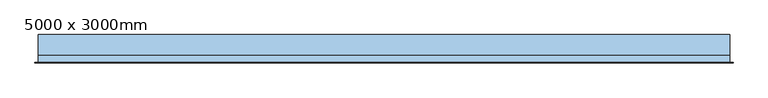
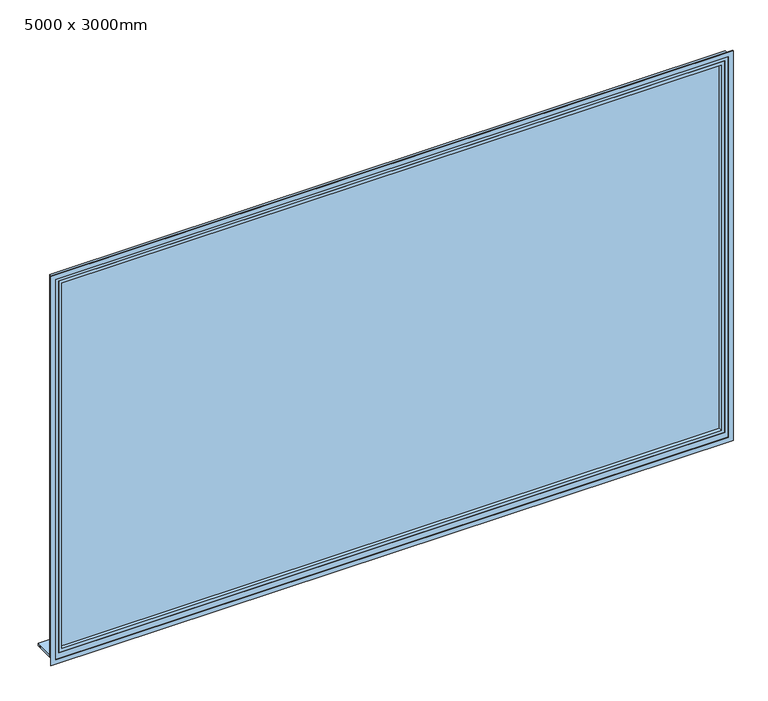
"""IFC4 building model written with IfcOpenShell, lengths in millimetres: window geometry, Ventana simple fija con cubrejuntas interior : 5000 x 3000mm."""

from ifc_helpers import new_model, si_unit, frame, origin, place, context, project, spatial, polyline, outline, extrude, faceted_brep, source, transform, mapped, element, save


def window_5000_x_3000mm_49c9fe68(model_context):
    return source(origin(), model_context, "Body", "SolidModel", [
        extrude(outline(polyline([(125.0, 920.0), (125.0, 900.0), (105.0, 900.0), (105.0, 910.0), (95.0, 910.0), (95.0, 900.0), (-25.0, 900.0), (-25.0, 920.0), (125.0, 920.0)])), frame((-2500.0, 0.0, 0.0), z_axis=(1.0, 0.0, 0.0), x_axis=(0.0, 1.0, 0.0)), (0.0, 0.0, 1.0), 5000.0),
        extrude(outline(polyline([(-2455.0, -49.0), (-2455.0, -35.0), (2455.0, -35.0), (2455.0, -49.0), (-2455.0, -49.0)])), frame((0.0, 0.0, 965.0), z_axis=(0.0, 0.0, 1.0), x_axis=(1.0, 0.0, 0.0)), (0.0, 0.0, 1.0), 2890.0),
        extrude(outline(polyline([(3865.0, -2465.0), (955.0, -2465.0), (955.0, 2465.0), (3865.0, 2465.0), (3865.0, -2465.0)]), holes=[polyline([(3840.0, 2440.0), (980.0, 2440.0), (980.0, -2440.0), (3840.0, -2440.0), (3840.0, 2440.0)])]), frame((0.0, -75.0, 0.0), z_axis=(0.0, 1.0, 0.0), x_axis=(0.0, 0.0, 1.0)), (0.0, 0.0, 1.0), 26.0),
        faceted_brep([(2500.0, -25.0, 3900.0), (2500.0, -75.0, 3900.0), (2500.0, -75.0, 900.0), (2500.0, -25.0, 900.0), (-2500.0, -75.0, 3900.0), (-2500.0, -75.0, 900.0), (-2465.0, -75.0, 3865.0), (2465.0, -75.0, 3865.0), (2465.0, -75.0, 955.0), (-2465.0, -75.0, 955.0), (-2500.0, -25.0, 900.0), (-2500.0, -25.0, 3900.0), (2440.0, -25.0, 3840.0), (-2440.0, -25.0, 3840.0), (-2440.0, -25.0, 980.0), (2440.0, -25.0, 980.0), (2440.0, -35.0, 3840.0), (2440.0, -35.0, 980.0), (-2440.0, -35.0, 980.0), (2465.0, -35.0, 3865.0), (-2465.0, -35.0, 3865.0), (-2465.0, -35.0, 955.0), (2465.0, -35.0, 955.0), (-2440.0, -35.0, 3840.0)], [[[0, 1, 2, 3]], [[2, 1, 4, 5], [6, 7, 8, 9]], [[5, 10, 3, 2]], [[10, 11, 0, 3], [12, 13, 14, 15]], [[16, 12, 15, 17]], [[17, 15, 14, 18]], [[19, 20, 21, 22], [23, 16, 17, 18]], [[7, 19, 22, 8]], [[8, 22, 21, 9]], [[13, 23, 18, 14]], [[20, 6, 9, 21]], [[4, 11, 10, 5]], [[11, 4, 1, 0]], [[23, 13, 12, 16]], [[6, 20, 19, 7]]]),
        extrude(outline(polyline([(3925.0, -2525.0), (875.0, -2525.0), (875.0, 2525.0), (3925.0, 2525.0), (3925.0, -2525.0)]), holes=[polyline([(3890.0, 2490.0), (910.0, 2490.0), (910.0, -2490.0), (3890.0, -2490.0), (3890.0, 2490.0)])]), frame((0.0, -80.0, 0.0), z_axis=(0.0, 1.0, 0.0), x_axis=(0.0, 0.0, 1.0)), (0.0, 0.0, 1.0), 5.0),
    ])


if __name__ == "__main__":
    model = new_model("IFC4")
    model_context = context("Model", 3, world=origin())
    ifc_project = project(units=[si_unit("LENGTHUNIT", "METRE", prefix="MILLI")], contexts=[model_context])
    site = spatial("IfcSite", under=ifc_project)
    building = spatial("IfcBuilding", under=site)
    placement = place(None, origin())
    window_5000_x_3000mm_shape = window_5000_x_3000mm_49c9fe68(model_context)
    element("IfcWindow", 1, ObjectType="Ventana simple fija con cubrejuntas interior : 5000 x 3000mm", at=placement, inside=building, context=model_context, shape_type="MappedRepresentation", body=[
        mapped(window_5000_x_3000mm_shape, transform((0.0, 0.0, 0.0), x_axis=(1.0, 0.0, 0.0), y_axis=(0.0, 1.0, 0.0), z_axis=(0.0, 0.0, 1.0))),
    ])
    save(model, "model.ifc")

# Revit data of these elements
# Type "Ventana simple fija con cubrejuntas interior : 5000 x 3000mm"
#   Type Mark = "41"
#   Construction Type Id = "GSP4R"
#   Analytic Construction = "1/8 en cristalera simple Pilkington"
#   Grosor de pared [instance default] = 0.20 m
#   W1 = 4.88 m
#   Visual Light Transmittance = 0.9
#   Anchura de cubrejuntas = 0.035 m
#   Grosor de cubrejuntas = 0.005 m
#   Solar Heat Gain Coefficient = 0.78
#   Grosor de antepecho = 0.02 m
#   Profundidad de antepecho [instance default] = 0.20 m
#   Rough Width = 5.00 m
#   Rough Height = 3.00 m
#   Height = 3.00 m
#   Heat Transfer Coefficient (U) = 3.6886 W/(m²·K)
#   Anchura de marco = 0.06 m
#   Grosor de marco = 0.05 m
#   Anchura de batiente de alzado = 0.50 m
#   Distancia entre antepecho y muro = 0.05 m
#   Altura de antepecho por defecto = 0.90 m
#   Width = 5.00 m
#   Define Thermal Properties by = 1
#   Material de antepecho = none
#   Material de cristalera = Vidrio
#   Material de estructura = none
#   Wall Closure = (empty or 0)
# Element 1 (IfcWindow, "Ventana simple fija con cubrejuntas interior : 5000 x 3000mm")
#   Grosor de pared = 0.15 m
#   Profundidad de antepecho = 0.15 m
#   Materials on its faces: "Vidrio"
# Materials
#   "Vidrio": class "Vidrio", colour RGB 245 245 243, transparency 1, Description = "Vidrio de cal sodada", Cost = 0
